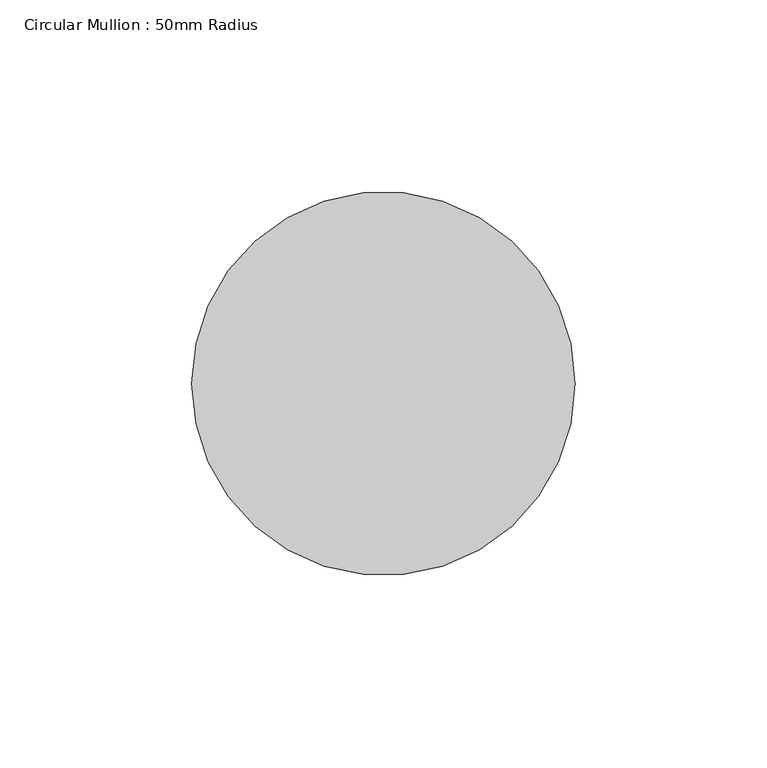
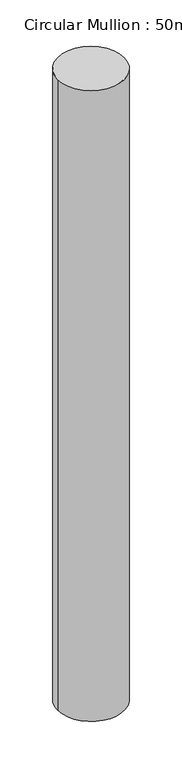
"""IFC4 building model written with IfcOpenShell, lengths in millimetres: member geometry, Circular Mullion : 50mm Radius."""

import ifcopenshell
import ifcopenshell.guid

model = None  # the IFC model being written
_history = None  # IfcOwnerHistory: only IFC2X3 demands one
_inside = {}  # id of a spatial element -> (the spatial element, [elements in it])
_under = {}  # id of a project, library or spatial element -> (it, [spatial elements below it])
_declared = {}  # id of a project -> (the project, [libraries it declares])
_typed = {}  # id of a type object -> (the type object, [elements of that type])
_made_of = {}  # id of a material, layer set ... -> (it, [elements and type objects made of it])


def new_model(schema):
    """Start an empty IFC model of exactly this schema.

    Asked for "IFC4X3", IfcOpenShell would pick the latest addendum, in which some entities
    have other attributes; the version numbers below select the first issue.
    IFC2X3 requires an IfcOwnerHistory on every rooted entity: one is made here for all.
    """
    global model, _history
    if schema == "IFC4X3":
        model = ifcopenshell.file(schema_version=(4, 3, 0, 0))
    else:
        model = ifcopenshell.file(schema=schema)
    _inside.clear()
    _under.clear()
    _declared.clear()
    _typed.clear()
    _made_of.clear()
    _history = None
    if model.schema == "IFC2X3":
        org = make("IfcOrganization", Name="unknown")
        user = make(
            "IfcPersonAndOrganization",
            ThePerson=make("IfcPerson", FamilyName="unknown"),
            TheOrganization=org,
        )
        app = make(
            "IfcApplication",
            ApplicationDeveloper=org,
            Version="unknown",
            ApplicationFullName="unknown",
            ApplicationIdentifier="unknown",
        )
        _history = make(
            "IfcOwnerHistory",
            OwningUser=user,
            OwningApplication=app,
            ChangeAction="ADDED",
            CreationDate=0,
        )
    return model


def make(cls, **values):
    """One entity of the class cls with the attributes given. An attribute that is None is left unset."""
    return model.create_entity(
        cls, **{name: value for name, value in values.items() if value is not None}
    )


def rooted(cls, **values):
    """An entity with a GlobalId (a new one), such as an element, a storey or a relation."""
    return make(cls, GlobalId=ifcopenshell.guid.new(), OwnerHistory=_history, **values)


def si_unit(unit_type, name, prefix=None):
    """IfcSIUnit, for example si_unit("LENGTHUNIT", "METRE", prefix="MILLI")."""
    return make("IfcSIUnit", UnitType=unit_type, Prefix=prefix, Name=name)


def assignment(units):
    """IfcUnitAssignment: the units of a project."""
    return None if units is None else make("IfcUnitAssignment", Units=units)


def point(xyz):
    """IfcCartesianPoint."""
    return None if xyz is None else make("IfcCartesianPoint", Coordinates=xyz)


def direction(xyz):
    """IfcDirection."""
    return None if xyz is None else make("IfcDirection", DirectionRatios=xyz)


def frame(location, z_axis=None, x_axis=None):
    """IfcAxis2Placement3D, a coordinate frame: its origin and axes. An axis left out is left unset."""
    return make(
        "IfcAxis2Placement3D",
        Location=point(location),
        Axis=direction(z_axis),
        RefDirection=direction(x_axis),
    )


def frame_2d(location, x_axis=None):
    """IfcAxis2Placement2D, a coordinate frame in the plane: its origin and x axis."""
    return make(
        "IfcAxis2Placement2D", Location=point(location), RefDirection=direction(x_axis)
    )


def origin():
    """The frame at (0, 0, 0) with its axes left unset."""
    return frame((0.0, 0.0, 0.0))


def origin_2d():
    """The frame at (0, 0) in the plane with its x axis left unset."""
    return frame_2d((0.0, 0.0))


def place(relative_to, where):
    """IfcLocalPlacement: puts the frame where relative to a parent placement (None: the world)."""
    return make(
        "IfcLocalPlacement", PlacementRelTo=relative_to, RelativePlacement=where
    )


def context(
    kind, dimensions, precision=None, world=None, true_north=None, identifier=None
):
    """IfcGeometricRepresentationContext, for example the 3D "Model" context."""
    return make(
        "IfcGeometricRepresentationContext",
        ContextIdentifier=identifier,
        ContextType=kind,
        CoordinateSpaceDimension=dimensions,
        Precision=precision,
        WorldCoordinateSystem=world,
        TrueNorth=true_north,
    )


def project(units=None, contexts=None):
    """IfcProject with its units and contexts."""
    return rooted(
        "IfcProject",
        Name="project",
        RepresentationContexts=contexts,
        UnitsInContext=assignment(units),
    )


def spatial(cls, under=None, at=None, **own):
    """A site, building, storey or space (cls), placed at a placement, below another one or the project."""
    s = rooted(cls, ObjectPlacement=at, **own)
    if under is not None:
        _under.setdefault(under.id(), (under, []))[1].append(s)
    return s


def circle_curve(where, radius):
    """IfcCircle in the frame where."""
    return make("IfcCircle", Position=where, Radius=radius)


def trimmed(basis, trim1, trim2, sense, master):
    """IfcTrimmedCurve: the piece of a basis curve between two trims."""
    return make(
        "IfcTrimmedCurve",
        BasisCurve=basis,
        Trim1=trim1,
        Trim2=trim2,
        SenseAgreement=sense,
        MasterRepresentation=master,
    )


def segment(curve, same_sense, transition):
    """IfcCompositeCurveSegment."""
    return make(
        "IfcCompositeCurveSegment",
        Transition=transition,
        SameSense=same_sense,
        ParentCurve=curve,
    )


def composite_curve(segments, self_intersect=None):
    """IfcCompositeCurve: segments joined end to end."""
    return make("IfcCompositeCurve", Segments=segments, SelfIntersect=self_intersect)


def outline(outer, holes=None, kind="AREA"):
    """IfcArbitraryClosedProfileDef: a profile drawn as a closed curve; with holes, ...WithVoids."""
    if holes is None:
        return make("IfcArbitraryClosedProfileDef", ProfileType=kind, OuterCurve=outer)
    return make(
        "IfcArbitraryProfileDefWithVoids",
        ProfileType=kind,
        OuterCurve=outer,
        InnerCurves=holes,
    )


def extrude(swept, where, along, depth):
    """IfcExtrudedAreaSolid: the profile swept, set in the frame where, extruded along a direction by depth."""
    return make(
        "IfcExtrudedAreaSolid",
        SweptArea=swept,
        Position=where,
        ExtrudedDirection=direction(along),
        Depth=depth,
    )


def shape(context_of_items, identifier, shape_type, items):
    """IfcShapeRepresentation: the items that make up one representation, for example the "Body"."""
    return make(
        "IfcShapeRepresentation",
        ContextOfItems=context_of_items,
        RepresentationIdentifier=identifier,
        RepresentationType=shape_type,
        Items=items,
    )


def source(mapping_origin, context_of_items, identifier, shape_type, items):
    """IfcRepresentationMap: a shape defined once, which mapped items show again and again."""
    return make(
        "IfcRepresentationMap",
        MappingOrigin=mapping_origin,
        MappedRepresentation=shape(context_of_items, identifier, shape_type, items),
    )


def transform(
    local_origin,
    x_axis=None,
    y_axis=None,
    z_axis=None,
    scale=None,
    scale2=None,
    scale3=None,
    uniform=True,
):
    """IfcCartesianTransformationOperator3D, or its non-uniform kind. x_axis, y_axis, z_axis: its Axis1, 2, 3."""
    if uniform:
        return make(
            "IfcCartesianTransformationOperator3D",
            Axis1=direction(x_axis),
            Axis2=direction(y_axis),
            LocalOrigin=point(local_origin),
            Scale=scale,
            Axis3=direction(z_axis),
        )
    return make(
        "IfcCartesianTransformationOperator3DnonUniform",
        Axis1=direction(x_axis),
        Axis2=direction(y_axis),
        LocalOrigin=point(local_origin),
        Scale=scale,
        Axis3=direction(z_axis),
        Scale2=scale2,
        Scale3=scale3,
    )


def mapped(mapping_source, mapping_target):
    """IfcMappedItem: shows the shape of a source again, moved by a transform."""
    return make(
        "IfcMappedItem", MappingSource=mapping_source, MappingTarget=mapping_target
    )


def made_of(thing, what):
    """Note that an element or type object is made of a material, layer set ...; save() writes the relation."""
    if what is not None:
        _made_of.setdefault(what.id(), (what, []))[1].append(thing)
    return thing


def element(
    cls,
    number,
    at=None,
    inside=None,
    cuts=None,
    type_object=None,
    material=None,
    context=None,
    identifier="Body",
    shape_type=None,
    held_by="IfcProductDefinitionShape",
    body=None,
    shapes=None,
    **own,
):
    """One element of the class cls, such as IfcWall. Its Tag is "e" and its number.

    at: its placement. inside: the storey or other place that contains it. cuts: it is an
    opening in that element (IfcRelVoidsElement). A single representation is given by context,
    identifier, shape_type and body (its items); several are given by shapes. held_by: the class
    of the entity that holds the representations. save() writes the other relations.
    """
    e = rooted(cls, Tag="e%d" % number, ObjectPlacement=at, **own)
    if body is not None:
        shapes = [shape(context, identifier, shape_type, body)]
    if shapes is not None:
        e.Representation = make(held_by, Representations=shapes)
    if inside is not None:
        _inside.setdefault(inside.id(), (inside, []))[1].append(e)
    if cuts is not None:
        rooted(
            "IfcRelVoidsElement", RelatingBuildingElement=cuts, RelatedOpeningElement=e
        )
    if type_object is not None:
        _typed.setdefault(type_object.id(), (type_object, []))[1].append(e)
    return made_of(e, material)


def aggregate(whole, parts):
    """IfcRelAggregates: a whole, such as a stair, and the parts it consists of."""
    return rooted("IfcRelAggregates", RelatingObject=whole, RelatedObjects=parts)


def save(model, path):
    """Write the relations noted so far, then the file.

    IfcRelAggregates (storeys below a building ...), IfcRelContainedInSpatialStructure (elements
    in a storey), IfcRelDefinesByType, IfcRelAssociatesMaterial and IfcRelDeclares: one each for
    every whole, place, type object, material and project.
    """
    for whole, parts in _under.values():
        aggregate(whole, parts)
    for where, things in _inside.values():
        rooted(
            "IfcRelContainedInSpatialStructure",
            RelatedElements=things,
            RelatingStructure=where,
        )
    for kind, things in _typed.values():
        rooted("IfcRelDefinesByType", RelatedObjects=things, RelatingType=kind)
    for what, things in _made_of.values():
        rooted("IfcRelAssociatesMaterial", RelatedObjects=things, RelatingMaterial=what)
    for by, libraries in _declared.values():
        rooted("IfcRelDeclares", RelatingContext=by, RelatedDefinitions=libraries)
    model.write(path)


def circular_mullion_50mm_radius_acc14b33(model_context):
    return source(origin(), model_context, "Body", "SweptSolid", [
        extrude(outline(composite_curve([segment(trimmed(circle_curve(origin_2d(), 50.0), [point((50.0, 0.0))], [point((-50.0, 0.0))], False, "CARTESIAN"), True, "CONTINUOUS"), segment(trimmed(circle_curve(origin_2d(), 50.0), [point((-50.0, 0.0))], [point((50.0, 0.0))], False, "CARTESIAN"), True, "CONTINUOUS")], self_intersect=False)), frame((0.0, 0.0, -1002.2516584), z_axis=(0.0, 0.0, 1.0), x_axis=(1.0, 0.0, 0.0)), (0.0, 0.0, 1.0), 1002.2516584),
    ])


if __name__ == "__main__":
    model = new_model("IFC4")
    model_context = context("Model", 3, world=origin())
    ifc_project = project(units=[si_unit("LENGTHUNIT", "METRE", prefix="MILLI")], contexts=[model_context])
    site = spatial("IfcSite", under=ifc_project)
    building = spatial("IfcBuilding", under=site)
    placement = place(None, origin())
    circular_mullion_50mm_radius_shape = circular_mullion_50mm_radius_acc14b33(model_context)
    element("IfcMember", 1, ObjectType="Circular Mullion : 50mm Radius", at=placement, inside=building, context=model_context, shape_type="MappedRepresentation", body=[
        mapped(circular_mullion_50mm_radius_shape, transform((0.0, 0.0, 0.0), x_axis=(1.0, 0.0, 0.0), y_axis=(0.0, 1.0, 0.0), z_axis=(0.0, 0.0, 1.0))),
    ])
    save(model, "model.ifc")

# Revit data of these elements
# Type "Circular Mullion : 50mm Radius"
#   built-in parameter 1007350 = 0.164042 (stored number, unit not read)
# Element 1 (IfcMember, "Circular Mullion : 50mm Radius")
#   Materials on its faces: "Aluminium"
# Materials
#   "Aluminium": class "Metal", colour RGB 247 247 247, transparency 0, Description = "Aluminium 6061", Cost = 0
